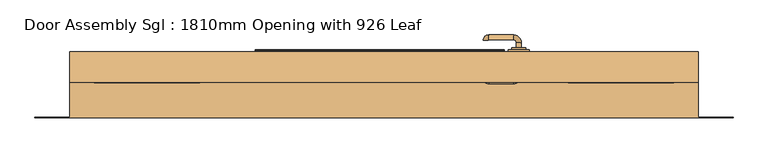
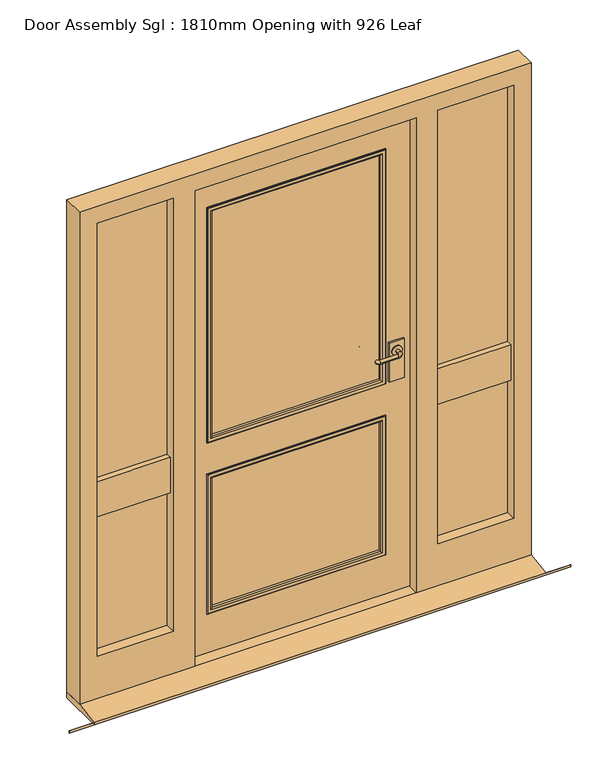
"""IFC4 building model written with IfcOpenShell, lengths in millimetres: door geometry, Door Assembly Sgl : 1810mm Opening with 926 Leaf."""

from ifc_helpers import new_model, si_unit, point, frame, frame_2d, origin, place, context, project, spatial, polyline, circle_curve, ellipse_curve, trimmed, segment, composite_curve, outline, extrude, faceted_brep, source, transform, mapped, element, save
from ifc_brep_helpers import plane_surface, cylinder_surface, revolved_surface, advanced_brep


def door_assembly_sgl_1810mm_opening_with_926_leaf_fb0b65bb(model_context):
    return source(origin(), model_context, "Body", "SolidModel", [
        extrude(outline(composite_curve([segment(trimmed(circle_curve(frame_2d((1050.0, 680.0)), 20.0), [point((1050.0, 700.0))], [point((1050.0, 660.0))], False, "CARTESIAN"), True, "CONTINUOUS"), segment(trimmed(circle_curve(frame_2d((1050.0, 680.0)), 20.0), [point((1050.0, 660.0))], [point((1050.0, 700.0))], False, "CARTESIAN"), True, "CONTINUOUS")], self_intersect=False)), frame((0.0, 28.75, 0.0), z_axis=(0.0, 1.0, 0.0), x_axis=(0.0, 0.0, 1.0)), (0.0, 0.0, 1.0), 4.5929895),
        advanced_brep(
        [(673.0, 33.3429895, 1050.0), (687.0, 33.3429895, 1050.0), (687.0, 48.75, 1050.0), (673.0, 48.75, 1050.0), (665.0, 70.75, 1050.0), (665.0, 56.75, 1050.0), (593.0, 70.75, 1050.0), (593.0, 56.75, 1050.0), (592.0, 55.75, 1050.0), (578.0, 55.75, 1050.0)],
        [
            (0, 1, circle_curve(frame((680.0, 33.3429895, 1050.0), z_axis=(0.0, -1.0, 0.0), x_axis=(1.0, 0.0, 0.0)), 7.0)),
            (1, 0, circle_curve(frame((680.0, 33.3429895, 1050.0), z_axis=(0.0, -1.0, 0.0), x_axis=(1.0, 0.0, 0.0)), 7.0)),
            (1, 2),
            (2, 3, circle_curve(frame((680.0, 48.75, 1050.0), z_axis=(0.0, -1.0, 0.0), x_axis=(1.0, 0.0, 0.0)), 7.0)),
            (3, 0),
            (3, 2, circle_curve(frame((680.0, 48.75, 1050.0), z_axis=(0.0, -1.0, 0.0), x_axis=(1.0, 0.0, 0.0)), 7.0)),
            (4, 5, circle_curve(frame((665.0, 63.75, 1050.0), z_axis=(1.0, 0.0, 0.0), x_axis=(0.0, 1.0, 0.0)), 7.0)),
            (5, 3, circle_curve(frame((665.0, 48.75, 1050.0), z_axis=(0.0, 0.0, -1.0), x_axis=(1.0, 0.0, 0.0)), 8.0)),
            (2, 4, circle_curve(frame((665.0, 48.75, 1050.0), z_axis=(0.0, 0.0, 1.0), x_axis=(1.0, 0.0, 0.0)), 22.0)),
            (5, 4, circle_curve(frame((665.0, 63.75, 1050.0), z_axis=(1.0, 0.0, 0.0), x_axis=(0.0, 1.0, 0.0)), 7.0)),
            (4, 6),
            (6, 7, circle_curve(frame((593.0, 63.75, 1050.0), z_axis=(1.0, 0.0, 0.0), x_axis=(0.0, 1.0, 0.0)), 7.0)),
            (7, 5),
            (7, 6, circle_curve(frame((593.0, 63.75, 1050.0), z_axis=(1.0, 0.0, 0.0), x_axis=(0.0, 1.0, 0.0)), 7.0)),
            (8, 9, circle_curve(frame((585.0, 55.75, 1050.0), z_axis=(0.0, -1.0, 0.0), x_axis=(-1.0, 0.0, 0.0)), 7.0)),
            (9, 8, circle_curve(frame((585.0, 55.75, 1050.0), z_axis=(0.0, -1.0, 0.0), x_axis=(-1.0, 0.0, 0.0)), 7.0)),
            (8, 7, circle_curve(frame((593.0, 55.75, 1050.0), z_axis=(0.0, 0.0, -1.0), x_axis=(0.0, 1.0, 0.0)), 1.0)),
            (6, 9, circle_curve(frame((593.0, 55.75, 1050.0), z_axis=(0.0, 0.0, 1.0), x_axis=(0.0, 1.0, 0.0)), 15.0)),
        ],
        [
            plane_surface(frame((680.0, 33.3429895, 1050.0), z_axis=(0.0, -1.0, 0.0), x_axis=(0.0, 0.0, 1.0))),
            cylinder_surface(frame((680.0, 33.3429895, 1050.0), z_axis=(0.0, -1.0, 0.0), x_axis=(1.0, 0.0, 0.0)), 7.0),
            revolved_surface(trimmed(ellipse_curve(frame((680.0, 48.75, 1050.0), z_axis=(0.0, 1.0, 0.0), x_axis=(1.0, 0.0, 0.0)), 7.0, 7.0), [point((673.0, 48.75, 1050.0))], [point((687.0, 48.75, 1050.0))], True, "CARTESIAN"), (665.0, 48.75, 1050.0), (0.0, 0.0, -1.0)),
            revolved_surface(trimmed(ellipse_curve(frame((680.0, 48.75, 1050.0), z_axis=(0.0, 1.0, 0.0), x_axis=(1.0, 0.0, 0.0)), 7.0, 7.0), [point((687.0, 48.75, 1050.0))], [point((673.0, 48.75, 1050.0))], True, "CARTESIAN"), (665.0, 48.75, 1050.0), (0.0, 0.0, -1.0)),
            cylinder_surface(frame((665.0, 63.75, 1050.0), z_axis=(1.0, 0.0, 0.0), x_axis=(0.0, 1.0, 0.0)), 7.0),
            plane_surface(frame((585.0, 55.75, 1050.0), z_axis=(0.0, -1.0, 0.0), x_axis=(0.0, 0.0, 1.0))),
            revolved_surface(trimmed(ellipse_curve(frame((593.0, 63.75, 1050.0), z_axis=(-1.0, 0.0, 0.0), x_axis=(0.0, 1.0, 0.0)), 7.0, 7.0), [point((593.0, 56.75, 1050.0))], [point((593.0, 70.75, 1050.0))], True, "CARTESIAN"), (593.0, 55.75, 1050.0), (0.0, 0.0, -1.0)),
            revolved_surface(trimmed(ellipse_curve(frame((593.0, 63.75, 1050.0), z_axis=(-1.0, 0.0, 0.0), x_axis=(0.0, 1.0, 0.0)), 7.0, 7.0), [point((593.0, 70.75, 1050.0))], [point((593.0, 56.75, 1050.0))], True, "CARTESIAN"), (593.0, 55.75, 1050.0), (0.0, 0.0, -1.0)),
        ],
        [
            (0, [[1, 2]]),
            (1, [[3, 4, 5, -2]]),
            (1, [[-5, 6, -3, -1]]),
            (2, [[7, 8, -4, 9]]),
            (3, [[10, -9, -6, -8]]),
            (4, [[11, 12, 13, -7]]),
            (4, [[-13, 14, -11, -10]]),
            (5, [[15, 16]]),
            (6, [[-15, 17, -12, 18]]),
            (7, [[-16, -18, -14, -17]]),
        ],
    ),
        extrude(outline(polyline([(650.0, 22.75), (650.0, 28.75), (710.0, 28.75), (710.0, 22.75), (650.0, 22.75)])), frame((0.0, 0.0, 925.0), z_axis=(0.0, 0.0, 1.0), x_axis=(1.0, 0.0, 0.0)), (0.0, 0.0, 1.0), 165.0),
        extrude(outline(composite_curve([segment(trimmed(circle_curve(frame_2d((1050.0, 680.0)), 20.0), [point((1050.0, 700.0))], [point((1050.0, 660.0))], False, "CARTESIAN"), True, "CONTINUOUS"), segment(trimmed(circle_curve(frame_2d((1050.0, 680.0)), 20.0), [point((1050.0, 660.0))], [point((1050.0, 700.0))], False, "CARTESIAN"), True, "CONTINUOUS")], self_intersect=False)), frame((0.0, -31.8429895, 0.0), z_axis=(0.0, 1.0, 0.0), x_axis=(0.0, 0.0, 1.0)), (0.0, 0.0, 1.0), 4.5929895),
        advanced_brep(
        [(673.0, -31.8429895, 1050.0), (687.0, -31.8429895, 1050.0), (673.0, -47.25, 1050.0), (687.0, -47.25, 1050.0), (665.0, -69.25, 1050.0), (665.0, -55.25, 1050.0), (593.0, -55.25, 1050.0), (593.0, -69.25, 1050.0), (592.0, -54.25, 1050.0), (578.0, -54.25, 1050.0)],
        [
            (0, 1, circle_curve(frame((680.0, -31.8429895, 1050.0), z_axis=(0.0, 1.0, 0.0), x_axis=(1.0, 0.0, 0.0)), 7.0)),
            (1, 0, circle_curve(frame((680.0, -31.8429895, 1050.0), z_axis=(0.0, 1.0, 0.0), x_axis=(1.0, 0.0, 0.0)), 7.0)),
            (0, 2),
            (2, 3, circle_curve(frame((680.0, -47.25, 1050.0), z_axis=(0.0, 1.0, 0.0), x_axis=(1.0, 0.0, 0.0)), 7.0)),
            (3, 1),
            (3, 2, circle_curve(frame((680.0, -47.25, 1050.0), z_axis=(0.0, 1.0, 0.0), x_axis=(1.0, 0.0, 0.0)), 7.0)),
            (4, 3, circle_curve(frame((665.0, -47.25, 1050.0), z_axis=(0.0, 0.0, 1.0), x_axis=(1.0, 0.0, 0.0)), 22.0)),
            (2, 5, circle_curve(frame((665.0, -47.25, 1050.0), z_axis=(0.0, 0.0, -1.0), x_axis=(1.0, 0.0, 0.0)), 8.0)),
            (5, 4, circle_curve(frame((665.0, -62.25, 1050.0), z_axis=(1.0, 0.0, 0.0), x_axis=(0.0, -1.0, 0.0)), 7.0)),
            (4, 5, circle_curve(frame((665.0, -62.25, 1050.0), z_axis=(1.0, 0.0, 0.0), x_axis=(0.0, -1.0, 0.0)), 7.0)),
            (5, 6),
            (6, 7, circle_curve(frame((593.0, -62.25, 1050.0), z_axis=(1.0, 0.0, 0.0), x_axis=(0.0, -1.0, 0.0)), 7.0)),
            (7, 4),
            (7, 6, circle_curve(frame((593.0, -62.25, 1050.0), z_axis=(1.0, 0.0, 0.0), x_axis=(0.0, -1.0, 0.0)), 7.0)),
            (8, 9, circle_curve(frame((585.0, -54.25, 1050.0), z_axis=(0.0, 1.0, 0.0), x_axis=(-1.0, 0.0, 0.0)), 7.0)),
            (9, 8, circle_curve(frame((585.0, -54.25, 1050.0), z_axis=(0.0, 1.0, 0.0), x_axis=(-1.0, 0.0, 0.0)), 7.0)),
            (9, 7, circle_curve(frame((593.0, -54.25, 1050.0), z_axis=(0.0, 0.0, 1.0), x_axis=(0.0, -1.0, 0.0)), 15.0)),
            (6, 8, circle_curve(frame((593.0, -54.25, 1050.0), z_axis=(0.0, 0.0, -1.0), x_axis=(0.0, -1.0, 0.0)), 1.0)),
        ],
        [
            plane_surface(frame((680.0, -31.8429895, 1050.0), z_axis=(0.0, 1.0, 0.0), x_axis=(0.0, 0.0, 1.0))),
            cylinder_surface(frame((680.0, -31.8429895, 1050.0), z_axis=(0.0, 1.0, 0.0), x_axis=(1.0, 0.0, 0.0)), 7.0),
            revolved_surface(trimmed(ellipse_curve(frame((680.0, -47.25, 1050.0), z_axis=(0.0, 1.0, 0.0), x_axis=(1.0, 0.0, 0.0)), 7.0, 7.0), [point((673.0, -47.25, 1050.0))], [point((687.0, -47.25, 1050.0))], True, "CARTESIAN"), (665.0, -47.25, 1050.0), (0.0, 0.0, -1.0)),
            revolved_surface(trimmed(ellipse_curve(frame((680.0, -47.25, 1050.0), z_axis=(0.0, 1.0, 0.0), x_axis=(1.0, 0.0, 0.0)), 7.0, 7.0), [point((687.0, -47.25, 1050.0))], [point((673.0, -47.25, 1050.0))], True, "CARTESIAN"), (665.0, -47.25, 1050.0), (0.0, 0.0, -1.0)),
            cylinder_surface(frame((665.0, -62.25, 1050.0), z_axis=(1.0, 0.0, 0.0), x_axis=(0.0, -1.0, 0.0)), 7.0),
            plane_surface(frame((585.0, -54.25, 1050.0), z_axis=(0.0, 1.0, 0.0), x_axis=(0.0, 0.0, 1.0))),
            revolved_surface(trimmed(ellipse_curve(frame((593.0, -62.25, 1050.0), z_axis=(1.0, 0.0, 0.0), x_axis=(0.0, -1.0, 0.0)), 7.0, 7.0), [point((593.0, -55.25, 1050.0))], [point((593.0, -69.25, 1050.0))], True, "CARTESIAN"), (593.0, -54.25, 1050.0), (0.0, 0.0, -1.0)),
            revolved_surface(trimmed(ellipse_curve(frame((593.0, -62.25, 1050.0), z_axis=(1.0, 0.0, 0.0), x_axis=(0.0, -1.0, 0.0)), 7.0, 7.0), [point((593.0, -69.25, 1050.0))], [point((593.0, -55.25, 1050.0))], True, "CARTESIAN"), (593.0, -54.25, 1050.0), (0.0, 0.0, -1.0)),
        ],
        [
            (0, [[1, 2]]),
            (1, [[-1, 3, 4, 5]]),
            (1, [[-2, -5, 6, -3]]),
            (2, [[7, -4, 8, 9]]),
            (3, [[-8, -6, -7, 10]]),
            (4, [[-9, 11, 12, 13]]),
            (4, [[-10, -13, 14, -11]]),
            (5, [[15, 16]]),
            (6, [[17, -12, 18, -16]]),
            (7, [[-18, -14, -17, -15]]),
        ],
    ),
        extrude(outline(polyline([(650.0, -21.25), (710.0, -21.25), (710.0, -27.25), (650.0, -27.25), (650.0, -21.25)])), frame((0.0, 0.0, 925.0), z_axis=(0.0, 0.0, 1.0), x_axis=(1.0, 0.0, 0.0)), (0.0, 0.0, 1.0), 165.0),
        extrude(outline(polyline([(1148.5, -0.25), (1148.5, -24.25), (800.0, -24.25), (800.0, -0.25), (1148.5, -0.25)])), frame((0.0, 0.0, 189.0), z_axis=(0.0, 0.0, 1.0), x_axis=(1.0, 0.0, 0.0)), (0.0, 0.0, 1.0), 605.0),
        extrude(outline(polyline([(1148.5, -0.25), (1148.5, -24.25), (800.0, -24.25), (800.0, -0.25), (1148.5, -0.25)])), frame((0.0, 0.0, 914.0), z_axis=(0.0, 0.0, 1.0), x_axis=(1.0, 0.0, 0.0)), (0.0, 0.0, 1.0), 1147.5),
        extrude(outline(polyline([(-216.0, -0.25), (-216.0, -24.25), (-564.5, -24.25), (-564.5, -0.25), (-216.0, -0.25)])), frame((0.0, 0.0, 189.0), z_axis=(0.0, 0.0, 1.0), x_axis=(1.0, 0.0, 0.0)), (0.0, 0.0, 1.0), 605.0),
        extrude(outline(polyline([(-216.0, -0.25), (-216.0, -24.25), (-564.5, -24.25), (-564.5, -0.25), (-216.0, -0.25)])), frame((0.0, 0.0, 914.0), z_axis=(0.0, 0.0, 1.0), x_axis=(1.0, 0.0, 0.0)), (0.0, 0.0, 1.0), 1147.5),
        faceted_brep([(1197.0, -66.25, 25.0), (736.0, -66.25, 25.0), (736.0, -24.25, 25.0), (758.0, -24.25, 25.0), (758.0, 22.75, 25.0), (1197.0, 22.75, 25.0), (1197.0, 22.75, 2110.0), (1197.0, -66.25, 2110.0), (758.0, 22.75, 2061.5), (-174.0, 22.75, 2061.5), (-174.0, 22.75, 25.0), (-613.0, 22.75, 25.0), (-613.0, 22.75, 2110.0), (1126.5, 22.75, 929.0), (1126.5, 22.75, 2039.5), (822.0, 22.75, 2039.5), (822.0, 22.75, 929.0), (822.0, 22.75, 779.0), (822.0, 22.75, 204.0), (1126.5, 22.75, 204.0), (1126.5, 22.75, 779.0), (-238.0, 22.75, 779.0), (-542.5, 22.75, 779.0), (-542.5, 22.75, 204.0), (-238.0, 22.75, 204.0), (-542.5, 22.75, 2039.5), (-542.5, 22.75, 929.0), (-238.0, 22.75, 929.0), (-238.0, 22.75, 2039.5), (758.0, -24.25, 2061.5), (-174.0, -24.25, 25.0), (-174.0, -24.25, 2061.5), (736.0, -24.25, 2039.5), (-152.0, -24.25, 2039.5), (-152.0, -24.25, 25.0), (-216.0, -24.25, 2061.5), (-216.0, -24.25, 914.0), (-564.5, -24.25, 914.0), (-564.5, -24.25, 2061.5), (-542.5, -24.25, 2039.5), (-542.5, -24.25, 929.0), (-238.0, -24.25, 929.0), (-238.0, -24.25, 2039.5), (1148.5, -24.25, 2061.5), (1148.5, -24.25, 914.0), (800.0, -24.25, 914.0), (800.0, -24.25, 2061.5), (822.0, -24.25, 2039.5), (822.0, -24.25, 929.0), (1126.5, -24.25, 929.0), (1126.5, -24.25, 2039.5), (1148.5, -24.25, 189.0), (800.0, -24.25, 189.0), (800.0, -24.25, 794.0), (1148.5, -24.25, 794.0), (1126.5, -24.25, 779.0), (822.0, -24.25, 779.0), (822.0, -24.25, 204.0), (1126.5, -24.25, 204.0), (-564.5, -24.25, 794.0), (-216.0, -24.25, 794.0), (-216.0, -24.25, 189.0), (-564.5, -24.25, 189.0), (-238.0, -24.25, 779.0), (-542.5, -24.25, 779.0), (-542.5, -24.25, 204.0), (-238.0, -24.25, 204.0), (736.0, -66.25, 2039.5), (-613.0, -66.25, 25.0), (-152.0, -66.25, 25.0), (-152.0, -66.25, 2039.5), (-613.0, -66.25, 2110.0), (-238.0, -66.25, 2039.5), (-238.0, -66.25, 204.0), (-542.5, -66.25, 204.0), (-542.5, -66.25, 2039.5), (1126.5, -66.25, 2039.5), (1126.5, -66.25, 204.0), (822.0, -66.25, 204.0), (822.0, -66.25, 2039.5), (-542.5, -47.25, 779.0), (-542.5, -47.25, 929.0), (-238.0, -47.25, 929.0), (-238.0, -47.25, 779.0), (822.0, -47.25, 779.0), (822.0, -47.25, 929.0), (1126.5, -47.25, 929.0), (1126.5, -47.25, 779.0), (822.0, -0.25, 929.0), (1126.5, -0.25, 929.0), (822.0, -0.25, 2039.5), (822.0, -0.25, 779.0), (822.0, -0.25, 204.0), (1126.5, -0.25, 2039.5), (1126.5, -0.25, 204.0), (1126.5, -0.25, 779.0), (-238.0, -0.25, 929.0), (-238.0, -0.25, 2039.5), (-238.0, -0.25, 204.0), (-238.0, -0.25, 779.0), (-542.5, -0.25, 204.0), (-542.5, -0.25, 2039.5), (-542.5, -0.25, 929.0), (-542.5, -0.25, 779.0), (1148.5, -0.25, 189.0), (1148.5, -0.25, 794.0), (1148.5, -0.25, 914.0), (1148.5, -0.25, 2061.5), (800.0, -0.25, 794.0), (800.0, -0.25, 189.0), (800.0, -0.25, 2061.5), (800.0, -0.25, 914.0), (-564.5, -0.25, 189.0), (-564.5, -0.25, 794.0), (-564.5, -0.25, 914.0), (-564.5, -0.25, 2061.5), (-216.0, -0.25, 914.0), (-216.0, -0.25, 2061.5), (-216.0, -0.25, 794.0), (-216.0, -0.25, 189.0)], [[[0, 1, 2, 3, 4, 5]], [[5, 6, 7, 0]], [[5, 4, 8, 9, 10, 11, 12, 6], [13, 14, 15, 16], [17, 18, 19, 20], [21, 22, 23, 24], [25, 26, 27, 28]], [[3, 29, 8, 4]], [[30, 31, 29, 3, 2, 32, 33, 34]], [[35, 36, 37, 38], [39, 40, 41, 42]], [[43, 44, 45, 46], [47, 48, 49, 50]], [[51, 52, 53, 54], [55, 56, 57, 58]], [[59, 60, 61, 62], [63, 64, 65, 66]], [[1, 67, 32, 2]], [[68, 69, 70, 67, 1, 0, 7, 71], [72, 73, 74, 75], [76, 77, 78, 79]], [[71, 12, 11, 68]], [[34, 33, 70, 69]], [[11, 10, 30, 34, 69, 68]], [[75, 74, 65, 64, 80, 81, 40, 39]], [[65, 74, 73, 66]], [[42, 41, 82, 83, 63, 66, 73, 72]], [[79, 78, 57, 56, 84, 85, 48, 47]], [[77, 58, 57, 78]], [[50, 49, 86, 87, 55, 58, 77, 76]], [[16, 88, 89, 13]], [[90, 88, 16, 15]], [[17, 91, 92, 18]], [[14, 13, 89, 93]], [[19, 94, 95, 20]], [[20, 95, 91, 17]], [[18, 92, 94, 19]], [[28, 27, 96, 97]], [[24, 98, 99, 21]], [[23, 100, 98, 24]], [[101, 102, 26, 25]], [[22, 103, 100, 23]], [[21, 99, 103, 22]], [[26, 102, 96, 27]], [[10, 9, 31, 30]], [[104, 51, 54, 105]], [[106, 44, 43, 107]], [[104, 105, 108, 109], [94, 92, 91, 95]], [[110, 111, 106, 107], [93, 89, 88, 90]], [[54, 53, 108, 105]], [[109, 52, 51, 104]], [[111, 45, 44, 106]], [[40, 81, 82, 41]], [[112, 113, 59, 62]], [[114, 115, 38, 37]], [[37, 36, 116, 114]], [[36, 35, 117, 116]], [[61, 60, 118, 119]], [[48, 85, 86, 49]], [[108, 53, 52, 109]], [[110, 46, 45, 111]], [[55, 87, 84, 56]], [[63, 83, 80, 64]], [[112, 62, 61, 119]], [[113, 118, 60, 59]], [[85, 84, 87, 86]], [[115, 114, 116, 117], [97, 96, 102, 101]], [[119, 118, 113, 112], [100, 103, 99, 98]], [[81, 80, 83, 82]], [[7, 6, 12, 71]], [[9, 8, 29, 31]], [[38, 115, 117, 35]], [[46, 110, 107, 43]], [[76, 79, 47, 50]], [[33, 32, 67, 70]], [[39, 42, 72, 75]], [[101, 25, 28, 97]], [[14, 93, 90, 15]]]),
        extrude(outline(polyline([(-71.0, -11.25), (-71.0, 12.75), (630.0, 12.75), (630.0, -11.25), (-71.0, -11.25)])), frame((0.0, 0.0, 929.0), z_axis=(0.0, 0.0, 1.0), x_axis=(1.0, 0.0, 0.0)), (0.0, 0.0, 1.0), 979.5),
        extrude(outline(polyline([(-71.0, -11.25), (-71.0, 12.75), (630.0, 12.75), (630.0, -11.25), (-71.0, -11.25)])), frame((0.0, 0.0, 204.0), z_axis=(0.0, 0.0, 1.0), x_axis=(1.0, 0.0, 0.0)), (0.0, 0.0, 1.0), 575.0),
        faceted_brep([(1297.0, -167.25, 0.0), (1297.0, -166.25, 0.0), (1297.0, -166.25, 9.2522001), (1297.0, -167.25, 9.0947221), (-713.0, -167.25, 9.0947221), (-713.0, -166.25, 9.2522001), (-713.0, -166.25, 0.0), (-713.0, -167.25, 0.0), (-613.0, -166.25, 0.0), (-613.0, 22.75, 0.0), (1197.0, 22.75, 0.0), (1197.0, -166.25, 0.0), (1197.0, -166.25, 9.2522001), (1197.0, -66.25, 25.0), (-613.0, -66.25, 25.0), (-613.0, -166.25, 9.2522001), (1197.0, 22.75, 25.0), (-613.0, 22.75, 25.0)], [[[0, 1, 2, 3]], [[4, 5, 6, 7]], [[7, 6, 8, 9, 10, 11, 1, 0]], [[3, 4, 7, 0]], [[3, 2, 12, 13, 14, 15, 5, 4]], [[14, 13, 16, 17]], [[17, 16, 10, 9]], [[15, 14, 17, 9, 8]], [[8, 6, 5, 15]], [[11, 10, 16, 13, 12]], [[12, 2, 1, 11]]]),
        extrude(outline(polyline([(29.0, -171.0), (29.0, 755.0), (2058.5, 755.0), (2058.5, -171.0), (29.0, -171.0)]), holes=[polyline([(1908.5, 630.0), (929.0, 630.0), (929.0, -71.0), (1908.5, -71.0), (1908.5, 630.0)]), polyline([(779.0, -71.0), (779.0, 630.0), (204.0, 630.0), (204.0, -71.0), (779.0, -71.0)])]), frame((0.0, -21.25, 0.0), z_axis=(0.0, 1.0, 0.0), x_axis=(0.0, 0.0, 1.0)), (0.0, 0.0, 1.0), 44.0),
        advanced_brep(
        [(630.0, 12.75, 779.0), (630.0, 12.75, 204.0), (630.0, 22.75, 204.0), (630.0, 22.75, 779.0), (618.0, 23.75, 767.0), (618.0, 23.75, 216.0), (618.0, 12.75, 216.0), (618.0, 12.75, 767.0), (623.0, 28.75, 772.0), (623.0, 28.75, 211.0), (638.0, 26.75, 787.0), (638.0, 26.75, 196.0), (636.0, 28.75, 198.0), (636.0, 28.75, 785.0), (638.0, 22.75, 787.0), (638.0, 22.75, 196.0), (-71.0, 12.75, 204.0), (-71.0, 22.75, 204.0), (-59.0, 23.75, 216.0), (-59.0, 12.75, 216.0), (-64.0, 28.75, 211.0), (-79.0, 26.75, 196.0), (-77.0, 28.75, 198.0), (-79.0, 22.75, 196.0), (-71.0, 12.75, 779.0), (-71.0, 22.75, 779.0), (-59.0, 23.75, 767.0), (-59.0, 12.75, 767.0), (-64.0, 28.75, 772.0), (-79.0, 26.75, 787.0), (-77.0, 28.75, 785.0), (-79.0, 22.75, 787.0)],
        [
            (0, 1),
            (1, 2),
            (2, 3),
            (3, 0),
            (4, 5),
            (5, 6),
            (6, 7),
            (7, 4),
            (8, 9),
            (9, 5, ellipse_curve(frame((623.0, 23.75, 211.0), z_axis=(0.7071067811865431, 0.0, 0.707106781186552), x_axis=(-0.7071067811865521, 0.0, 0.7071067811865429)), 7.0710678, 5.0)),
            (4, 8, ellipse_curve(frame((623.0, 23.75, 772.0), z_axis=(0.707106781186552, 0.0, -0.707106781186543), x_axis=(0.7071067811865429, 0.0, 0.707106781186552)), 7.0710678, 5.0)),
            (10, 11),
            (11, 12, ellipse_curve(frame((636.0, 26.75, 198.0), z_axis=(0.7071067811865431, 0.0, 0.707106781186552), x_axis=(-0.7071067811865521, 0.0, 0.7071067811865429)), 2.8284271, 2.0)),
            (12, 13),
            (13, 10, ellipse_curve(frame((636.0, 26.75, 785.0), z_axis=(0.707106781186552, 0.0, -0.707106781186543), x_axis=(0.7071067811865429, 0.0, 0.707106781186552)), 2.8284271, 2.0)),
            (14, 15),
            (15, 11),
            (10, 14),
            (1, 16),
            (16, 17),
            (17, 2),
            (5, 18),
            (18, 19),
            (19, 6),
            (9, 20),
            (20, 18, ellipse_curve(frame((-64.0, 23.75, 211.0), z_axis=(0.707106781186552, 0.0, -0.7071067811865431), x_axis=(0.7071067811865429, 0.0, 0.707106781186552)), 7.0710678, 5.0)),
            (11, 21),
            (21, 22, ellipse_curve(frame((-77.0, 26.75, 198.0), z_axis=(0.707106781186552, 0.0, -0.7071067811865431), x_axis=(0.7071067811865429, 0.0, 0.707106781186552)), 2.8284271, 2.0)),
            (22, 12),
            (15, 23),
            (23, 21),
            (16, 24),
            (24, 25),
            (25, 17),
            (18, 26),
            (26, 27),
            (27, 19),
            (20, 28),
            (28, 26, ellipse_curve(frame((-64.0, 23.75, 772.0), z_axis=(-0.707106781186543, 0.0, -0.7071067811865519), x_axis=(0.7071067811865517, 0.0, -0.7071067811865432)), 7.0710678, 5.0)),
            (21, 29),
            (29, 30, ellipse_curve(frame((-77.0, 26.75, 785.0), z_axis=(-0.707106781186543, 0.0, -0.7071067811865519), x_axis=(0.7071067811865517, 0.0, -0.7071067811865432)), 2.8284271, 2.0)),
            (30, 22),
            (23, 31),
            (31, 29),
            (14, 31),
            (25, 3),
            (24, 0),
            (27, 7),
            (26, 4),
            (28, 8),
            (30, 13),
            (29, 10),
        ],
        [
            plane_surface(frame((630.0, 22.75, 779.0), z_axis=(1.0, 0.0, 0.0), x_axis=(0.0, 0.0, -1.0))),
            plane_surface(frame((618.0, 12.75, 767.0), z_axis=(-1.0, 0.0, 0.0), x_axis=(0.0, 0.0, -1.0))),
            cylinder_surface(frame((623.0, 23.75, 779.0), z_axis=(0.0, 0.0, 1.0), x_axis=(1.0, 0.0, 0.0)), 5.0),
            cylinder_surface(frame((636.0, 26.75, 779.0), z_axis=(0.0, 0.0, 1.0), x_axis=(1.0, 0.0, 0.0)), 2.0),
            plane_surface(frame((638.0, 26.75, 787.0), z_axis=(1.0, 0.0, 0.0), x_axis=(0.0, 0.0, -1.0))),
            plane_surface(frame((630.0, 22.75, 204.0), z_axis=(0.0, 0.0, -1.0), x_axis=(-1.0, 0.0, 0.0))),
            plane_surface(frame((618.0, 12.75, 216.0), z_axis=(0.0, 0.0, 1.0), x_axis=(-1.0, 0.0, 0.0))),
            cylinder_surface(frame((630.0, 23.75, 211.0), z_axis=(1.0, 0.0, 0.0), x_axis=(0.0, 0.0, -1.0)), 5.0),
            cylinder_surface(frame((630.0, 26.75, 198.0), z_axis=(1.0, 0.0, 0.0), x_axis=(0.0, 0.0, -1.0)), 2.0),
            plane_surface(frame((638.0, 26.75, 196.0), z_axis=(0.0, 0.0, -1.0), x_axis=(-1.0, 0.0, 0.0))),
            plane_surface(frame((-71.0, 22.75, 204.0), z_axis=(-1.0, 0.0, 0.0), x_axis=(0.0, 0.0, 1.0))),
            plane_surface(frame((-59.0, 12.75, 216.0), z_axis=(1.0, 0.0, 0.0), x_axis=(0.0, 0.0, 1.0))),
            cylinder_surface(frame((-64.0, 23.75, 204.0), z_axis=(0.0, 0.0, -1.0), x_axis=(-1.0, 0.0, 0.0)), 5.0),
            cylinder_surface(frame((-77.0, 26.75, 204.0), z_axis=(0.0, 0.0, -1.0), x_axis=(-1.0, 0.0, 0.0)), 2.0),
            plane_surface(frame((-79.0, 26.75, 196.0), z_axis=(-1.0, 0.0, 0.0), x_axis=(0.0, 0.0, 1.0))),
            plane_surface(frame((-79.0, 22.75, 787.0), z_axis=(0.0, -1.0, 0.0), x_axis=(1.0, 0.0, 0.0))),
            plane_surface(frame((-71.0, 22.75, 779.0), z_axis=(0.0, 0.0, 1.0), x_axis=(1.0, 0.0, 0.0))),
            plane_surface(frame((-71.0, 12.75, 779.0), z_axis=(0.0, -1.0, 0.0), x_axis=(1.0, 0.0, 0.0))),
            plane_surface(frame((-59.0, 12.75, 767.0), z_axis=(0.0, 0.0, -1.0), x_axis=(1.0, 0.0, 0.0))),
            cylinder_surface(frame((-71.0, 23.75, 772.0), z_axis=(-1.0, 0.0, 0.0), x_axis=(0.0, 0.0, 1.0)), 5.0),
            plane_surface(frame((-64.0, 28.75, 772.0), z_axis=(0.0, 1.0, 0.0), x_axis=(1.0, 0.0, 0.0))),
            cylinder_surface(frame((-71.0, 26.75, 785.0), z_axis=(-1.0, 0.0, 0.0), x_axis=(0.0, 0.0, 1.0)), 2.0),
            plane_surface(frame((-79.0, 26.75, 787.0), z_axis=(0.0, 0.0, 1.0), x_axis=(1.0, 0.0, 0.0))),
        ],
        [
            (0, [[1, 2, 3, 4]]),
            (1, [[5, 6, 7, 8]]),
            (2, [[9, 10, -5, 11]]),
            (3, [[12, 13, 14, 15]]),
            (4, [[16, 17, -12, 18]]),
            (5, [[19, 20, 21, -2]]),
            (6, [[22, 23, 24, -6]]),
            (7, [[25, 26, -22, -10]]),
            (8, [[27, 28, 29, -13]]),
            (9, [[30, 31, -27, -17]]),
            (10, [[32, 33, 34, -20]]),
            (11, [[35, 36, 37, -23]]),
            (12, [[38, 39, -35, -26]]),
            (13, [[40, 41, 42, -28]]),
            (14, [[43, 44, -40, -31]]),
            (15, [[-16, 45, -43, -30], [-3, -21, -34, 46]]),
            (16, [[47, -4, -46, -33]]),
            (17, [[-1, -47, -32, -19], [-7, -24, -37, 48]]),
            (18, [[49, -8, -48, -36]]),
            (19, [[50, -11, -49, -39]]),
            (20, [[-14, -29, -42, 51], [-9, -50, -38, -25]]),
            (21, [[52, -15, -51, -41]]),
            (22, [[-45, -18, -52, -44]]),
        ],
    ),
        advanced_brep(
        [(-71.0, -11.25, 779.0), (-71.0, -11.25, 204.0), (-71.0, -21.25, 204.0), (-71.0, -21.25, 779.0), (-59.0, -22.25, 767.0), (-59.0, -22.25, 216.0), (-59.0, -11.25, 216.0), (-59.0, -11.25, 767.0), (-64.0, -27.25, 772.0), (-64.0, -27.25, 211.0), (-79.0, -25.25, 787.0), (-79.0, -25.25, 196.0), (-77.0, -27.25, 198.0), (-77.0, -27.25, 785.0), (-79.0, -21.25, 787.0), (-79.0, -21.25, 196.0), (630.0, -11.25, 204.0), (630.0, -21.25, 204.0), (618.0, -22.25, 216.0), (618.0, -11.25, 216.0), (623.0, -27.25, 211.0), (638.0, -25.25, 196.0), (636.0, -27.25, 198.0), (638.0, -21.25, 196.0), (630.0, -11.25, 779.0), (630.0, -21.25, 779.0), (618.0, -22.25, 767.0), (618.0, -11.25, 767.0), (623.0, -27.25, 772.0), (638.0, -25.25, 787.0), (636.0, -27.25, 785.0), (638.0, -21.25, 787.0)],
        [
            (0, 1),
            (1, 2),
            (2, 3),
            (3, 0),
            (4, 5),
            (5, 6),
            (6, 7),
            (7, 4),
            (8, 9),
            (9, 5, ellipse_curve(frame((-64.0, -22.25, 211.0), z_axis=(-0.7071067811865475, 0.0, 0.7071067811865475), x_axis=(0.7071067811865474, 0.0, 0.7071067811865476)), 7.0710678, 5.0)),
            (4, 8, ellipse_curve(frame((-64.0, -22.25, 772.0), z_axis=(-0.7071067811865475, 0.0, -0.7071067811865475), x_axis=(-0.7071067811865474, 0.0, 0.7071067811865477)), 7.0710678, 5.0)),
            (10, 11),
            (11, 12, ellipse_curve(frame((-77.0, -25.25, 198.0), z_axis=(-0.7071067811865475, 0.0, 0.7071067811865475), x_axis=(0.7071067811865474, 0.0, 0.7071067811865476)), 2.8284271, 2.0)),
            (12, 13),
            (13, 10, ellipse_curve(frame((-77.0, -25.25, 785.0), z_axis=(-0.7071067811865475, 0.0, -0.7071067811865475), x_axis=(-0.7071067811865474, 0.0, 0.7071067811865477)), 2.8284271, 2.0)),
            (14, 15),
            (15, 11),
            (10, 14),
            (1, 16),
            (16, 17),
            (17, 2),
            (5, 18),
            (18, 19),
            (19, 6),
            (9, 20),
            (20, 18, ellipse_curve(frame((623.0, -22.25, 211.0), z_axis=(-0.7071067811865475, 0.0, -0.7071067811865475), x_axis=(-0.7071067811865476, 0.0, 0.7071067811865474)), 7.0710678, 5.0)),
            (11, 21),
            (21, 22, ellipse_curve(frame((636.0, -25.25, 198.0), z_axis=(-0.7071067811865475, 0.0, -0.7071067811865475), x_axis=(-0.7071067811865476, 0.0, 0.7071067811865474)), 2.8284271, 2.0)),
            (22, 12),
            (15, 23),
            (23, 21),
            (16, 24),
            (24, 25),
            (25, 17),
            (18, 26),
            (26, 27),
            (27, 19),
            (20, 28),
            (28, 26, ellipse_curve(frame((623.0, -22.25, 772.0), z_axis=(0.7071067811865475, 0.0, -0.7071067811865475), x_axis=(-0.7071067811865474, 0.0, -0.7071067811865477)), 7.0710678, 5.0)),
            (21, 29),
            (29, 30, ellipse_curve(frame((636.0, -25.25, 785.0), z_axis=(0.7071067811865475, 0.0, -0.7071067811865475), x_axis=(-0.7071067811865474, 0.0, -0.7071067811865477)), 2.8284271, 2.0)),
            (30, 22),
            (23, 31),
            (31, 29),
            (14, 31),
            (25, 3),
            (24, 0),
            (27, 7),
            (26, 4),
            (28, 8),
            (30, 13),
            (29, 10),
        ],
        [
            plane_surface(frame((-71.0, -21.25, 779.0), z_axis=(-1.0, 0.0, 0.0), x_axis=(0.0, 0.0, -1.0))),
            plane_surface(frame((-59.0, -11.25, 767.0), z_axis=(1.0, 0.0, 0.0), x_axis=(0.0, 0.0, -1.0))),
            cylinder_surface(frame((-64.0, -22.25, 779.0), z_axis=(0.0, 0.0, 1.0), x_axis=(-1.0, 0.0, 0.0)), 5.0),
            cylinder_surface(frame((-77.0, -25.25, 779.0), z_axis=(0.0, 0.0, 1.0), x_axis=(-1.0, 0.0, 0.0)), 2.0),
            plane_surface(frame((-79.0, -25.25, 787.0), z_axis=(-1.0, 0.0, 0.0), x_axis=(0.0, 0.0, -1.0))),
            plane_surface(frame((-71.0, -21.25, 204.0), z_axis=(0.0, 0.0, -1.0), x_axis=(1.0, 0.0, 0.0))),
            plane_surface(frame((-59.0, -11.25, 216.0), z_axis=(0.0, 0.0, 1.0), x_axis=(1.0, 0.0, 0.0))),
            cylinder_surface(frame((-71.0, -22.25, 211.0), z_axis=(-1.0, 0.0, 0.0), x_axis=(0.0, 0.0, -1.0)), 5.0),
            cylinder_surface(frame((-71.0, -25.25, 198.0), z_axis=(-1.0, 0.0, 0.0), x_axis=(0.0, 0.0, -1.0)), 2.0),
            plane_surface(frame((-79.0, -25.25, 196.0), z_axis=(0.0, 0.0, -1.0), x_axis=(1.0, 0.0, 0.0))),
            plane_surface(frame((630.0, -21.25, 204.0), z_axis=(1.0, 0.0, 0.0), x_axis=(0.0, 0.0, 1.0))),
            plane_surface(frame((618.0, -11.25, 216.0), z_axis=(-1.0, 0.0, 0.0), x_axis=(0.0, 0.0, 1.0))),
            cylinder_surface(frame((623.0, -22.25, 204.0), z_axis=(0.0, 0.0, -1.0), x_axis=(1.0, 0.0, 0.0)), 5.0),
            cylinder_surface(frame((636.0, -25.25, 204.0), z_axis=(0.0, 0.0, -1.0), x_axis=(1.0, 0.0, 0.0)), 2.0),
            plane_surface(frame((638.0, -25.25, 196.0), z_axis=(1.0, 0.0, 0.0), x_axis=(0.0, 0.0, 1.0))),
            plane_surface(frame((638.0, -21.25, 787.0), z_axis=(0.0, 1.0, 0.0), x_axis=(-1.0, 0.0, 0.0))),
            plane_surface(frame((630.0, -21.25, 779.0), z_axis=(0.0, 0.0, 1.0), x_axis=(-1.0, 0.0, 0.0))),
            plane_surface(frame((630.0, -11.25, 779.0), z_axis=(0.0, 1.0, 0.0), x_axis=(-1.0, 0.0, 0.0))),
            plane_surface(frame((618.0, -11.25, 767.0), z_axis=(0.0, 0.0, -1.0), x_axis=(-1.0, 0.0, 0.0))),
            cylinder_surface(frame((630.0, -22.25, 772.0), z_axis=(1.0, 0.0, 0.0), x_axis=(0.0, 0.0, 1.0)), 5.0),
            plane_surface(frame((623.0, -27.25, 772.0), z_axis=(0.0, -1.0, 0.0), x_axis=(-1.0, 0.0, 0.0))),
            cylinder_surface(frame((630.0, -25.25, 785.0), z_axis=(1.0, 0.0, 0.0), x_axis=(0.0, 0.0, 1.0)), 2.0),
            plane_surface(frame((638.0, -25.25, 787.0), z_axis=(0.0, 0.0, 1.0), x_axis=(-1.0, 0.0, 0.0))),
        ],
        [
            (0, [[1, 2, 3, 4]]),
            (1, [[5, 6, 7, 8]]),
            (2, [[9, 10, -5, 11]]),
            (3, [[12, 13, 14, 15]]),
            (4, [[16, 17, -12, 18]]),
            (5, [[19, 20, 21, -2]]),
            (6, [[22, 23, 24, -6]]),
            (7, [[25, 26, -22, -10]]),
            (8, [[27, 28, 29, -13]]),
            (9, [[30, 31, -27, -17]]),
            (10, [[32, 33, 34, -20]]),
            (11, [[35, 36, 37, -23]]),
            (12, [[38, 39, -35, -26]]),
            (13, [[40, 41, 42, -28]]),
            (14, [[43, 44, -40, -31]]),
            (15, [[-16, 45, -43, -30], [-3, -21, -34, 46]]),
            (16, [[47, -4, -46, -33]]),
            (17, [[-1, -47, -32, -19], [-7, -24, -37, 48]]),
            (18, [[49, -8, -48, -36]]),
            (19, [[50, -11, -49, -39]]),
            (20, [[-14, -29, -42, 51], [-9, -50, -38, -25]]),
            (21, [[52, -15, -51, -41]]),
            (22, [[-45, -18, -52, -44]]),
        ],
    ),
        advanced_brep(
        [(-79.0, -25.25, 921.0), (-79.0, -25.25, 1916.5), (-79.0, -21.25, 1916.5), (-79.0, -21.25, 921.0), (-77.0, -27.25, 923.0), (-77.0, -27.25, 1914.5), (-59.0, -22.25, 941.0), (-59.0, -22.25, 1896.5), (-64.0, -27.25, 1901.5), (-64.0, -27.25, 936.0), (-59.0, -11.25, 941.0), (-59.0, -11.25, 1896.5), (-71.0, -21.25, 929.0), (-71.0, -21.25, 1908.5), (-71.0, -11.25, 1908.5), (-71.0, -11.25, 929.0), (638.0, -25.25, 1916.5), (638.0, -21.25, 1916.5), (636.0, -27.25, 1914.5), (618.0, -22.25, 1896.5), (623.0, -27.25, 1901.5), (618.0, -11.25, 1896.5), (630.0, -21.25, 1908.5), (630.0, -11.25, 1908.5), (638.0, -25.25, 921.0), (638.0, -21.25, 921.0), (636.0, -27.25, 923.0), (618.0, -22.25, 941.0), (623.0, -27.25, 936.0), (618.0, -11.25, 941.0), (630.0, -21.25, 929.0), (630.0, -11.25, 929.0)],
        [
            (0, 1),
            (1, 2),
            (2, 3),
            (3, 0),
            (4, 5),
            (5, 1, ellipse_curve(frame((-77.0, -25.25, 1914.5), z_axis=(-0.7071067811865476, 0.0, -0.7071067811865474), x_axis=(0.7071067811865474, 0.0, -0.7071067811865478)), 2.8284271, 2.0)),
            (0, 4, ellipse_curve(frame((-77.0, -25.25, 923.0), z_axis=(-0.7071067811865475, 0.0, 0.7071067811865476), x_axis=(-0.7071067811865475, 0.0, -0.7071067811865475)), 2.8284271, 2.0)),
            (6, 7),
            (7, 8, ellipse_curve(frame((-64.0, -22.25, 1901.5), z_axis=(-0.7071067811865476, 0.0, -0.7071067811865474), x_axis=(0.7071067811865474, 0.0, -0.7071067811865478)), 7.0710678, 5.0)),
            (8, 9),
            (9, 6, ellipse_curve(frame((-64.0, -22.25, 936.0), z_axis=(-0.7071067811865475, 0.0, 0.7071067811865476), x_axis=(-0.7071067811865475, 0.0, -0.7071067811865475)), 7.0710678, 5.0)),
            (10, 11),
            (11, 7),
            (6, 10),
            (12, 13),
            (13, 14),
            (14, 15),
            (15, 12),
            (1, 16),
            (16, 17),
            (17, 2),
            (5, 18),
            (18, 16, ellipse_curve(frame((636.0, -25.25, 1914.5), z_axis=(-0.7071067811865475, 0.0, 0.7071067811865476), x_axis=(-0.7071067811865475, 0.0, -0.7071067811865475)), 2.8284271, 2.0)),
            (7, 19),
            (19, 20, ellipse_curve(frame((623.0, -22.25, 1901.5), z_axis=(-0.7071067811865475, 0.0, 0.7071067811865476), x_axis=(-0.7071067811865475, 0.0, -0.7071067811865475)), 7.0710678, 5.0)),
            (20, 8),
            (11, 21),
            (21, 19),
            (13, 22),
            (22, 23),
            (23, 14),
            (16, 24),
            (24, 25),
            (25, 17),
            (18, 26),
            (26, 24, ellipse_curve(frame((636.0, -25.25, 923.0), z_axis=(0.7071067811865476, 0.0, 0.7071067811865475), x_axis=(-0.7071067811865475, 0.0, 0.7071067811865475)), 2.8284271, 2.0)),
            (19, 27),
            (27, 28, ellipse_curve(frame((623.0, -22.25, 936.0), z_axis=(0.7071067811865476, 0.0, 0.7071067811865475), x_axis=(-0.7071067811865475, 0.0, 0.7071067811865475)), 7.0710678, 5.0)),
            (28, 20),
            (21, 29),
            (29, 27),
            (22, 30),
            (30, 31),
            (31, 23),
            (24, 0),
            (3, 25),
            (26, 4),
            (28, 9),
            (27, 6),
            (29, 10),
            (31, 15),
            (30, 12),
        ],
        [
            plane_surface(frame((-79.0, -21.25, 921.0), z_axis=(-1.0, 0.0, 0.0), x_axis=(0.0, 0.0, 1.0))),
            cylinder_surface(frame((-77.0, -25.25, 929.0), z_axis=(0.0, 0.0, -1.0), x_axis=(-1.0, 0.0, 0.0)), 2.0),
            cylinder_surface(frame((-64.0, -22.25, 929.0), z_axis=(0.0, 0.0, -1.0), x_axis=(-1.0, 0.0, 0.0)), 5.0),
            plane_surface(frame((-59.0, -22.25, 941.0), z_axis=(1.0, 0.0, 0.0), x_axis=(0.0, 0.0, 1.0))),
            plane_surface(frame((-71.0, -11.25, 929.0), z_axis=(-1.0, 0.0, 0.0), x_axis=(0.0, 0.0, 1.0))),
            plane_surface(frame((-79.0, -21.25, 1916.5), z_axis=(0.0, 0.0, 1.0), x_axis=(1.0, 0.0, 0.0))),
            cylinder_surface(frame((-71.0, -25.25, 1914.5), z_axis=(-1.0, 0.0, 0.0), x_axis=(0.0, 0.0, 1.0)), 2.0),
            cylinder_surface(frame((-71.0, -22.25, 1901.5), z_axis=(-1.0, 0.0, 0.0), x_axis=(0.0, 0.0, 1.0)), 5.0),
            plane_surface(frame((-59.0, -22.25, 1896.5), z_axis=(0.0, 0.0, -1.0), x_axis=(1.0, 0.0, 0.0))),
            plane_surface(frame((-71.0, -11.25, 1908.5), z_axis=(0.0, 0.0, 1.0), x_axis=(1.0, 0.0, 0.0))),
            plane_surface(frame((638.0, -21.25, 1916.5), z_axis=(1.0, 0.0, 0.0), x_axis=(0.0, 0.0, -1.0))),
            cylinder_surface(frame((636.0, -25.25, 1908.5), z_axis=(0.0, 0.0, 1.0), x_axis=(1.0, 0.0, 0.0)), 2.0),
            cylinder_surface(frame((623.0, -22.25, 1908.5), z_axis=(0.0, 0.0, 1.0), x_axis=(1.0, 0.0, 0.0)), 5.0),
            plane_surface(frame((618.0, -22.25, 1896.5), z_axis=(-1.0, 0.0, 0.0), x_axis=(0.0, 0.0, -1.0))),
            plane_surface(frame((630.0, -11.25, 1908.5), z_axis=(1.0, 0.0, 0.0), x_axis=(0.0, 0.0, -1.0))),
            plane_surface(frame((638.0, -21.25, 921.0), z_axis=(0.0, 0.0, -1.0), x_axis=(-1.0, 0.0, 0.0))),
            cylinder_surface(frame((630.0, -25.25, 923.0), z_axis=(1.0, 0.0, 0.0), x_axis=(0.0, 0.0, -1.0)), 2.0),
            plane_surface(frame((636.0, -27.25, 923.0), z_axis=(0.0, -1.0, 0.0), x_axis=(-1.0, 0.0, 0.0))),
            cylinder_surface(frame((630.0, -22.25, 936.0), z_axis=(1.0, 0.0, 0.0), x_axis=(0.0, 0.0, -1.0)), 5.0),
            plane_surface(frame((618.0, -22.25, 941.0), z_axis=(0.0, 0.0, 1.0), x_axis=(-1.0, 0.0, 0.0))),
            plane_surface(frame((618.0, -11.25, 941.0), z_axis=(0.0, 1.0, 0.0), x_axis=(-1.0, 0.0, 0.0))),
            plane_surface(frame((630.0, -11.25, 929.0), z_axis=(0.0, 0.0, -1.0), x_axis=(-1.0, 0.0, 0.0))),
            plane_surface(frame((630.0, -21.25, 929.0), z_axis=(0.0, 1.0, 0.0), x_axis=(-1.0, 0.0, 0.0))),
        ],
        [
            (0, [[1, 2, 3, 4]]),
            (1, [[5, 6, -1, 7]]),
            (2, [[8, 9, 10, 11]]),
            (3, [[12, 13, -8, 14]]),
            (4, [[15, 16, 17, 18]]),
            (5, [[19, 20, 21, -2]]),
            (6, [[22, 23, -19, -6]]),
            (7, [[24, 25, 26, -9]]),
            (8, [[27, 28, -24, -13]]),
            (9, [[29, 30, 31, -16]]),
            (10, [[32, 33, 34, -20]]),
            (11, [[35, 36, -32, -23]]),
            (12, [[37, 38, 39, -25]]),
            (13, [[40, 41, -37, -28]]),
            (14, [[42, 43, 44, -30]]),
            (15, [[45, -4, 46, -33]]),
            (16, [[47, -7, -45, -36]]),
            (17, [[-5, -47, -35, -22], [-10, -26, -39, 48]]),
            (18, [[49, -11, -48, -38]]),
            (19, [[50, -14, -49, -41]]),
            (20, [[-17, -31, -44, 51], [-12, -50, -40, -27]]),
            (21, [[52, -18, -51, -43]]),
            (22, [[-3, -21, -34, -46], [-15, -52, -42, -29]]),
        ],
    ),
        advanced_brep(
        [(630.0, 12.75, 1908.5), (630.0, 12.75, 929.0), (630.0, 22.75, 929.0), (630.0, 22.75, 1908.5), (618.0, 23.75, 1896.5), (618.0, 23.75, 941.0), (618.0, 12.75, 941.0), (618.0, 12.75, 1896.5), (623.0, 28.75, 1901.5), (623.0, 28.75, 936.0), (638.0, 26.75, 1916.5), (638.0, 26.75, 921.0), (636.0, 28.75, 923.0), (636.0, 28.75, 1914.5), (638.0, 22.75, 1916.5), (638.0, 22.75, 921.0), (-71.0, 12.75, 929.0), (-71.0, 22.75, 929.0), (-59.0, 23.75, 941.0), (-59.0, 12.75, 941.0), (-64.0, 28.75, 936.0), (-79.0, 26.75, 921.0), (-77.0, 28.75, 923.0), (-79.0, 22.75, 921.0), (-71.0, 12.75, 1908.5), (-71.0, 22.75, 1908.5), (-59.0, 23.75, 1896.5), (-59.0, 12.75, 1896.5), (-64.0, 28.75, 1901.5), (-79.0, 26.75, 1916.5), (-77.0, 28.75, 1914.5), (-79.0, 22.75, 1916.5)],
        [
            (0, 1),
            (1, 2),
            (2, 3),
            (3, 0),
            (4, 5),
            (5, 6),
            (6, 7),
            (7, 4),
            (8, 9),
            (9, 5, ellipse_curve(frame((623.0, 23.75, 936.0), z_axis=(0.7071067811865475, 0.0, 0.7071067811865475), x_axis=(-0.7071067811865474, 0.0, 0.7071067811865476)), 7.0710678, 5.0)),
            (4, 8, ellipse_curve(frame((623.0, 23.75, 1901.5), z_axis=(0.7071067811865475, 0.0, -0.7071067811865475), x_axis=(0.7071067811865474, 0.0, 0.7071067811865476)), 7.0710678, 5.0)),
            (10, 11),
            (11, 12, ellipse_curve(frame((636.0, 26.75, 923.0), z_axis=(0.7071067811865475, 0.0, 0.7071067811865475), x_axis=(-0.7071067811865474, 0.0, 0.7071067811865476)), 2.8284271, 2.0)),
            (12, 13),
            (13, 10, ellipse_curve(frame((636.0, 26.75, 1914.5), z_axis=(0.7071067811865475, 0.0, -0.7071067811865475), x_axis=(0.7071067811865474, 0.0, 0.7071067811865476)), 2.8284271, 2.0)),
            (14, 15),
            (15, 11),
            (10, 14),
            (1, 16),
            (16, 17),
            (17, 2),
            (5, 18),
            (18, 19),
            (19, 6),
            (9, 20),
            (20, 18, ellipse_curve(frame((-64.0, 23.75, 936.0), z_axis=(0.7071067811865475, 0.0, -0.7071067811865475), x_axis=(0.7071067811865476, 0.0, 0.7071067811865474)), 7.0710678, 5.0)),
            (11, 21),
            (21, 22, ellipse_curve(frame((-77.0, 26.75, 923.0), z_axis=(0.7071067811865475, 0.0, -0.7071067811865475), x_axis=(0.7071067811865476, 0.0, 0.7071067811865474)), 2.8284271, 2.0)),
            (22, 12),
            (15, 23),
            (23, 21),
            (16, 24),
            (24, 25),
            (25, 17),
            (18, 26),
            (26, 27),
            (27, 19),
            (20, 28),
            (28, 26, ellipse_curve(frame((-64.0, 23.75, 1901.5), z_axis=(-0.7071067811865475, 0.0, -0.7071067811865475), x_axis=(0.7071067811865474, 0.0, -0.7071067811865476)), 7.0710678, 5.0)),
            (21, 29),
            (29, 30, ellipse_curve(frame((-77.0, 26.75, 1914.5), z_axis=(-0.7071067811865475, 0.0, -0.7071067811865475), x_axis=(0.7071067811865474, 0.0, -0.7071067811865476)), 2.8284271, 2.0)),
            (30, 22),
            (23, 31),
            (31, 29),
            (14, 31),
            (25, 3),
            (24, 0),
            (27, 7),
            (26, 4),
            (28, 8),
            (30, 13),
            (29, 10),
        ],
        [
            plane_surface(frame((630.0, 22.75, 1908.5), z_axis=(1.0, 0.0, 0.0), x_axis=(0.0, 0.0, -1.0))),
            plane_surface(frame((618.0, 12.75, 1896.5), z_axis=(-1.0, 0.0, 0.0), x_axis=(0.0, 0.0, -1.0))),
            cylinder_surface(frame((623.0, 23.75, 1908.5), z_axis=(0.0, 0.0, 1.0), x_axis=(1.0, 0.0, 0.0)), 5.0),
            cylinder_surface(frame((636.0, 26.75, 1908.5), z_axis=(0.0, 0.0, 1.0), x_axis=(1.0, 0.0, 0.0)), 2.0),
            plane_surface(frame((638.0, 26.75, 1916.5), z_axis=(1.0, 0.0, 0.0), x_axis=(0.0, 0.0, -1.0))),
            plane_surface(frame((630.0, 22.75, 929.0), z_axis=(0.0, 0.0, -1.0), x_axis=(-1.0, 0.0, 0.0))),
            plane_surface(frame((618.0, 12.75, 941.0), z_axis=(0.0, 0.0, 1.0), x_axis=(-1.0, 0.0, 0.0))),
            cylinder_surface(frame((630.0, 23.75, 936.0), z_axis=(1.0, 0.0, 0.0), x_axis=(0.0, 0.0, -1.0)), 5.0),
            cylinder_surface(frame((630.0, 26.75, 923.0), z_axis=(1.0, 0.0, 0.0), x_axis=(0.0, 0.0, -1.0)), 2.0),
            plane_surface(frame((638.0, 26.75, 921.0), z_axis=(0.0, 0.0, -1.0), x_axis=(-1.0, 0.0, 0.0))),
            plane_surface(frame((-71.0, 22.75, 929.0), z_axis=(-1.0, 0.0, 0.0), x_axis=(0.0, 0.0, 1.0))),
            plane_surface(frame((-59.0, 12.75, 941.0), z_axis=(1.0, 0.0, 0.0), x_axis=(0.0, 0.0, 1.0))),
            cylinder_surface(frame((-64.0, 23.75, 929.0), z_axis=(0.0, 0.0, -1.0), x_axis=(-1.0, 0.0, 0.0)), 5.0),
            cylinder_surface(frame((-77.0, 26.75, 929.0), z_axis=(0.0, 0.0, -1.0), x_axis=(-1.0, 0.0, 0.0)), 2.0),
            plane_surface(frame((-79.0, 26.75, 921.0), z_axis=(-1.0, 0.0, 0.0), x_axis=(0.0, 0.0, 1.0))),
            plane_surface(frame((-79.0, 22.75, 1916.5), z_axis=(0.0, -1.0, 0.0), x_axis=(1.0, 0.0, 0.0))),
            plane_surface(frame((-71.0, 22.75, 1908.5), z_axis=(0.0, 0.0, 1.0), x_axis=(1.0, 0.0, 0.0))),
            plane_surface(frame((-71.0, 12.75, 1908.5), z_axis=(0.0, -1.0, 0.0), x_axis=(1.0, 0.0, 0.0))),
            plane_surface(frame((-59.0, 12.75, 1896.5), z_axis=(0.0, 0.0, -1.0), x_axis=(1.0, 0.0, 0.0))),
            cylinder_surface(frame((-71.0, 23.75, 1901.5), z_axis=(-1.0, 0.0, 0.0), x_axis=(0.0, 0.0, 1.0)), 5.0),
            plane_surface(frame((-64.0, 28.75, 1901.5), z_axis=(0.0, 1.0, 0.0), x_axis=(1.0, 0.0, 0.0))),
            cylinder_surface(frame((-71.0, 26.75, 1914.5), z_axis=(-1.0, 0.0, 0.0), x_axis=(0.0, 0.0, 1.0)), 2.0),
            plane_surface(frame((-79.0, 26.75, 1916.5), z_axis=(0.0, 0.0, 1.0), x_axis=(1.0, 0.0, 0.0))),
        ],
        [
            (0, [[1, 2, 3, 4]]),
            (1, [[5, 6, 7, 8]]),
            (2, [[9, 10, -5, 11]]),
            (3, [[12, 13, 14, 15]]),
            (4, [[16, 17, -12, 18]]),
            (5, [[19, 20, 21, -2]]),
            (6, [[22, 23, 24, -6]]),
            (7, [[25, 26, -22, -10]]),
            (8, [[27, 28, 29, -13]]),
            (9, [[30, 31, -27, -17]]),
            (10, [[32, 33, 34, -20]]),
            (11, [[35, 36, 37, -23]]),
            (12, [[38, 39, -35, -26]]),
            (13, [[40, 41, 42, -28]]),
            (14, [[43, 44, -40, -31]]),
            (15, [[-16, 45, -43, -30], [-3, -21, -34, 46]]),
            (16, [[47, -4, -46, -33]]),
            (17, [[-1, -47, -32, -19], [-7, -24, -37, 48]]),
            (18, [[49, -8, -48, -36]]),
            (19, [[50, -11, -49, -39]]),
            (20, [[-14, -29, -42, 51], [-9, -50, -38, -25]]),
            (21, [[52, -15, -51, -41]]),
            (22, [[-45, -18, -52, -44]]),
        ],
    ),
    ])


if __name__ == "__main__":
    model = new_model("IFC4")
    model_context = context("Model", 3, world=origin())
    ifc_project = project(units=[si_unit("LENGTHUNIT", "METRE", prefix="MILLI")], contexts=[model_context])
    site = spatial("IfcSite", under=ifc_project)
    building = spatial("IfcBuilding", under=site)
    placement = place(None, origin())
    door_assembly_sgl_1810mm_opening_with_926_leaf_shape = door_assembly_sgl_1810mm_opening_with_926_leaf_fb0b65bb(model_context)
    element("IfcDoor", 1, ObjectType="Door Assembly Sgl : 1810mm Opening with 926 Leaf", at=placement, inside=building, context=model_context, shape_type="MappedRepresentation", body=[
        mapped(door_assembly_sgl_1810mm_opening_with_926_leaf_shape, transform((0.0, 0.0, 0.0), x_axis=(1.0, 0.0, 0.0), y_axis=(0.0, 1.0, 0.0), z_axis=(0.0, 0.0, 1.0))),
    ])
    save(model, "model.ifc")

# Revit data of these elements
# Type "Door Assembly Sgl : 1810mm Opening with 926 Leaf"
#   Type Mark = "64"
#   Type Comments = "External Single"
#   Operation = "SingleSwingLeft"
#   Construction Type Id = "GSP4R"
#   Keynote = "L10"
#   Analytic Construction = "1/8 in Pilkington single glazing"
#   Wrap Layers (Int) from Ext = 215 mm
#   Wrap Layers (Ext) from Ext = 100 mm
#   Visual Light Transmittance = 0.9
#   Top of Lock Rail = 900 mm
#   Thickness = 44 mm
#   Stile Top Rail = 150 mm
#   Stile Shutting = 125 mm
#   Stile Lock Rail = 150 mm
#   Stile Hanging = 100 mm
#   Stile Bottom Rail = 175 mm
#   Solar Heat Gain Coefficient = 0.78
#   Rough Width = 1810 mm
#   Rough Height = 2110 mm
#   O/A Frame Width = 64 mm
#   Heat Transfer Coefficient (U) = 3.6886 W/(m²·K)
#   Handle Z Distance = 1050 mm
#   Glazing Thickness = 24 mm
#   FrameWidth = 42 mm
#   FrameOffset - External = 100 mm
#   FrameDepth = 89 mm
#   Door Panel Width = 926 mm
#   Door Panel Thickness = 44 mm
#   Door Panel Height = 2029.5 mm
#   Cill Thickness = 25 mm
#   Cill Projection = 1 mm
#   Handle X Distance = 75 mm
#   Height = 2110 mm
#   Structural Tolerance = 6.5 mm
#   Tolerance = 3 mm
#   Undercut = 4 mm
#   Width = 1810 mm
#   Cill Extension = 100 mm
#   Cavity Closer Width = 100 mm
#   Cavity Closer Offset from Ext = 100 mm
#   Cavity Closer Depth = 95 mm
#   Vis - Ironmongery = yes
#   Vis - Cavity Closers = no
#   Function = 1
#   Material Glass = Glass
#   Handle Style = element 425020
#   Material Door = Door - Panel
#   Material Frame = Door - Frame/Mullion
#   Material Ironmongery = Door - Handle
#   Wall Closure = (empty or 0)
# Element 1 (IfcDoor, "Door Assembly Sgl : 1810mm Opening with 926 Leaf")
#   Materials on its faces: "Door - Panel", "Door - Frame/Mullion", "Door - Handle", "Glass"
# Materials
#   "Glass": class "Glass", colour RGB 0 128 192, transparency 0.9, Description = "Soda Lime Glass", Cost = 0
#   "Door - Panel": class "Wood", colour RGB 210 159 95, transparency 0, Keynote = "L20"
#   "Door - Frame/Mullion": class "Wood", colour RGB 212 179 113, transparency 0, Keynote = "L20"
#   "Door - Handle": class "Miscellaneous", colour RGB 0 0 0, transparency 0, Keynote = "P21"
